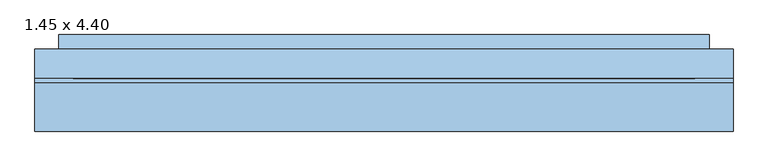
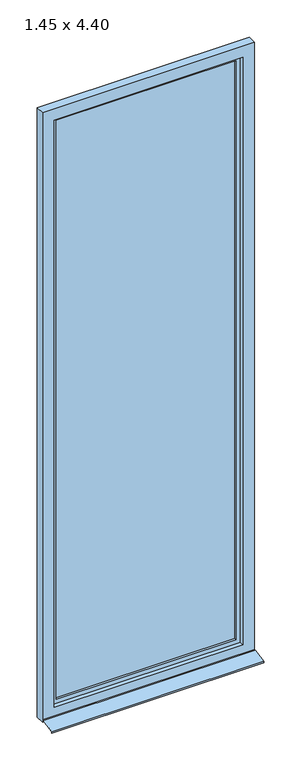
"""IFC4 building model written with IfcOpenShell, lengths in millimetres: window geometry, Fenstertür 1-flg : 1.45 x 4.40."""

from ifc_helpers import new_model, si_unit, frame, origin, place, context, project, spatial, polyline, outline, extrude, faceted_brep, source, transform, mapped, element, save


def window_1_45_x_4_40_705c903d(model_context):
    return source(origin(), model_context, "Body", "SolidModel", [
        extrude(outline(polyline([(4400.0, 725.0), (4400.0, -725.0), (0.0, -725.0), (0.0, 725.0), (4400.0, 725.0)]), holes=[polyline([(4320.0, 645.0), (80.0, 645.0), (80.0, -645.0), (4320.0, -645.0), (4320.0, 645.0)])]), frame((0.0, -95.0, 0.0), z_axis=(0.0, 1.0, 0.0), x_axis=(0.0, 0.0, 1.0)), (0.0, 0.0, 1.0), 60.0),
        faceted_brep([(675.0, -35.0, 4350.0), (675.0, -35.0, 50.0), (675.0, -5.0, 50.0), (675.0, -5.0, 4350.0), (-675.0, -5.0, 50.0), (-675.0, -5.0, 4350.0), (615.0, -5.0, 110.0), (615.0, -5.0, 4290.0), (-615.0, -5.0, 4290.0), (-615.0, -5.0, 110.0), (-675.0, -35.0, 50.0), (-675.0, -35.0, 4350.0), (645.0, -35.0, 4320.0), (645.0, -35.0, 80.0), (-645.0, -35.0, 80.0), (-645.0, -35.0, 4320.0), (645.0, -65.0, 4320.0), (645.0, -65.0, 80.0), (-645.0, -65.0, 80.0), (-645.0, -65.0, 4320.0), (615.0, -65.0, 4290.0), (615.0, -65.0, 110.0), (-615.0, -65.0, 110.0), (-615.0, -65.0, 4290.0)], [[[0, 1, 2, 3]], [[3, 2, 4, 5], [6, 7, 8, 9]], [[1, 10, 4, 2]], [[1, 0, 11, 10], [12, 13, 14, 15]], [[16, 17, 13, 12]], [[17, 18, 14, 13]], [[17, 16, 19, 18], [20, 21, 22, 23]], [[7, 6, 21, 20]], [[6, 9, 22, 21]], [[10, 11, 5, 4]], [[18, 19, 15, 14]], [[9, 8, 23, 22]], [[11, 0, 3, 5]], [[19, 16, 12, 15]], [[8, 7, 20, 23]]]),
        extrude(outline(polyline([(-105.0221543, 20.0), (-95.0, 20.0), (-95.0, 18.0), (-104.8240723, 18.0), (-203.0, -1.6395366), (-203.0, -10.0), (-205.0, -10.0), (-205.0, 0.0), (-105.0221543, 20.0)])), frame((-725.0, 0.0, 0.0), z_axis=(1.0, 0.0, 0.0), x_axis=(0.0, 1.0, 0.0)), (0.0, 0.0, 1.0), 1450.0),
        extrude(outline(polyline([(615.0, -20.0), (615.0, -50.0), (-615.0, -50.0), (-615.0, -20.0), (615.0, -20.0)])), frame((0.0, 0.0, 110.0), z_axis=(0.0, 0.0, 1.0), x_axis=(1.0, 0.0, 0.0)), (0.0, 0.0, 1.0), 4180.0),
    ])


if __name__ == "__main__":
    model = new_model("IFC4")
    model_context = context("Model", 3, world=origin())
    ifc_project = project(units=[si_unit("LENGTHUNIT", "METRE", prefix="MILLI")], contexts=[model_context])
    site = spatial("IfcSite", under=ifc_project)
    building = spatial("IfcBuilding", under=site)
    placement = place(None, origin())
    window_1_45_x_4_40_shape = window_1_45_x_4_40_705c903d(model_context)
    element("IfcWindow", 1, ObjectType="Fenstertür 1-flg : 1.45 x 4.40", at=placement, inside=building, context=model_context, shape_type="MappedRepresentation", body=[
        mapped(window_1_45_x_4_40_shape, transform((0.0, 0.0, 0.0), x_axis=(1.0, 0.0, 0.0), y_axis=(0.0, 1.0, 0.0), z_axis=(0.0, 0.0, 1.0))),
    ])
    save(model, "model.ifc")

# Revit data of these elements
# Type "Fenstertür 1-flg : 1.45 x 4.40"
#   Type Mark = "57"
#   Operation = "SinglePanel"
#   Construction Type Id = "GSP4R"
#   Keynote = "16.05.01"
#   Analytic Construction = "1/8 Zoll Pilkington-Verglasung einfach"
#   Visual Light Transmittance = 0.9
#   Thermal Resistance (R) = 0.1491 (m²·K)/W
#   Solar Heat Gain Coefficient = 0.86
#   Rough Width = 1.450 m
#   Rough Height = 4.400 m
#   Heat Transfer Coefficient (U) = 6.7069 W/(m²·K)
#   Rahmentiefe = 0.060 m
#   Rahmenhöhe - unten = 0.080 m
#   Rahmenhöhe - oben = 0.080 m
#   Rahmenbreite = 0.080 m
#   Height = 4.400 m
#   Tiefe Flügel = 0.060 m
#   Flügelbreite = 0.060 m
#   Einbautiefe (von außen) [instance default] = 0.080 m
#   Width = 1.450 m
#   Kippflügel [instance default] = yes
#   Drehflügel im Grundriss darstellen [instance default] = yes
#   Drehflügel 1 [instance default] = yes
#   Rahmen 1 [instance default] = none
#   Glas [instance default] = none
#   Flügel [instance default] = none
#   Fensterbank Außenseite [instance default] = none
#   Wall Closure = (empty or 0)
# Element 1 (IfcWindow, "Fenstertür 1-flg : 1.45 x 4.40")
#   Materials on its faces: "Kunststoff - Weiß", "Glas"
# Materials
#   "Kunststoff - Weiß": class "Kunststoff", colour RGB 249 249 249, transparency 0, Cost = 0
#   "Glas": class "Glas", colour RGB 0 0 255, transparency 0.75, Comments = "Render-Darstellung nicht aktualisiert ", Cost = 0
